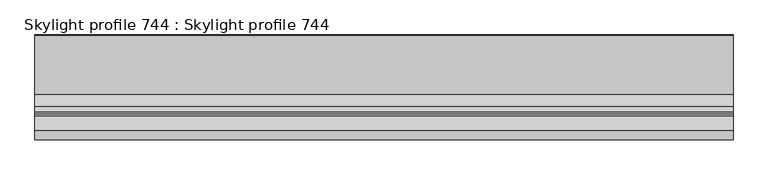
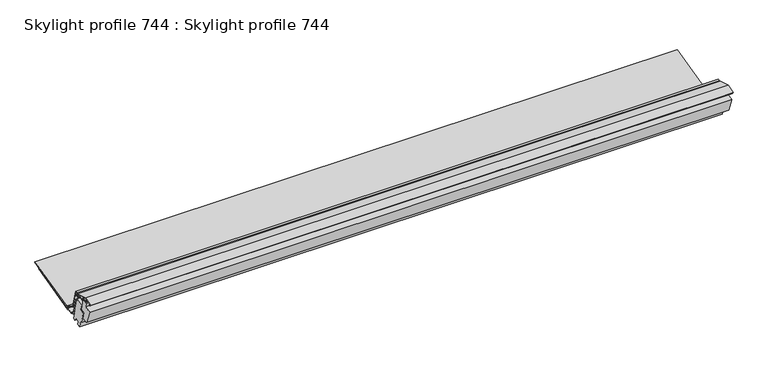
"""IFC4 building model written with IfcOpenShell, lengths in millimetres: proxy geometry, Skylight profile 744 : Skylight profile 744."""

from ifc_helpers import new_model, si_unit, frame, origin, place, context, project, spatial, polyline, outline, extrude, source, transform, mapped, element, save


def skylight_profile_744_skylight_profile_744_1989968f(model_context):
    return source(origin(), model_context, "Body", "SweptSolid", [
        extrude(outline(polyline([(10096.2573508, 43922.7064483), (10097.532491, 43917.6093806), (10110.1927133, 43920.7766051), (10113.4657593, 43918.8134908), (10115.0114469, 43912.6349746), (10131.6084885, 43916.7870784), (10137.0317176, 43914.2634297), (10139.0616447, 43910.1098329), (10137.264753, 43909.2316641), (10135.5458023, 43912.7489473), (10131.4068102, 43914.6749883), (10114.2973907, 43910.3947022), (10113.3713061, 43910.9501485), (10111.7266049, 43917.5244479), (10109.8744364, 43918.6353454), (10096.8184351, 43915.3691083), (10095.8923497, 43915.9245567), (10094.3171441, 43922.2210642), (10096.2573508, 43922.7064483)])), frame((3694.2883192, 0.0, 0.0), z_axis=(1.0, 0.0, 0.0), x_axis=(0.0, 1.0, 0.0)), (0.0, 0.0, 1.0), 2000.0),
        extrude(outline(polyline([(10079.242927, 43916.6221925), (10076.0312489, 43915.6964689), (10070.3693011, 43922.1990472), (10096.8276113, 43930.3081292), (10140.044925, 43917.228695), (10143.8105165, 43907.064565), (10138.5810742, 43903.9384198), (10137.5548647, 43905.6550718), (10141.3576537, 43907.9283678), (10138.5146506, 43915.6022359), (10096.8312865, 43928.2174303), (10073.9003145, 43921.1894255), (10076.7023802, 43917.9713366), (10078.6890046, 43918.5439547), (10079.242927, 43916.6221925)])), frame((3694.2883192, 0.0, 0.0), z_axis=(1.0, 0.0, 0.0), x_axis=(0.0, 1.0, 0.0)), (0.0, 0.0, 1.0), 2000.0),
        extrude(outline(polyline([(10145.985181, 43916.620671), (10151.5395078, 43918.0102043), (10165.844379, 43860.8299046), (10200.5304181, 43840.4836582), (10370.7180003, 43881.8704659), (10371.1905938, 43879.927104), (10200.2165946, 43838.3490527), (10164.1080064, 43859.5297424), (10150.0846852, 43915.5846135), (10148.412109, 43915.1661829), (10150.5052335, 43906.8238331), (10148.5653616, 43906.3371125), (10145.985181, 43916.620671)])), frame((3694.2883192, 0.0, 0.0), z_axis=(1.0, 0.0, 0.0), x_axis=(0.0, 1.0, 0.0)), (0.0, 0.0, 1.0), 2000.0),
        extrude(outline(polyline([(10194.6501599, 43830.8599821), (10192.6334981, 43834.9408699), (10176.4964673, 43831.2231764), (10162.6063897, 43836.4479074), (10149.394688, 43889.2597364), (10151.3348974, 43889.74511), (10164.2920903, 43837.9506423), (10176.6356497, 43833.3076316), (10193.7257878, 43837.2449047), (10195.7260908, 43833.1971203), (10350.9375941, 43872.6548936), (10351.4303591, 43870.7165482), (10194.6501599, 43830.8599821)])), frame((3694.2883192, 0.0, 0.0), z_axis=(1.0, 0.0, 0.0), x_axis=(0.0, 1.0, 0.0)), (0.0, 0.0, 1.0), 2000.0),
        extrude(outline(polyline([(10156.2334346, 43820.5271586), (10149.2528163, 43831.0794667), (10137.2155603, 43828.0680904), (10139.1867552, 43817.2760241), (10129.8324627, 43814.9063018), (10124.2729101, 43837.129283), (10118.717164, 43835.7393946), (10109.6828906, 43871.8517409), (10123.5722524, 43875.3264609), (10119.6342367, 43891.0677364), (10144.6350908, 43897.3222331), (10155.6384747, 43853.338722), (10154.7125446, 43853.1070809), (10162.472623, 43822.0880246), (10156.2334346, 43820.5271586)])), frame((3694.2883192, 0.0, 0.0), z_axis=(1.0, 0.0, 0.0), x_axis=(0.0, 1.0, 0.0)), (0.0, 0.0, 1.0), 2000.0),
        extrude(outline(polyline([(10119.2566248, 43878.3792301), (10105.7016033, 43874.747173), (10110.7413045, 43854.6029382), (10094.4955764, 43850.538723), (10092.6158882, 43851.5362563), (10076.658138, 43895.2717658), (10097.9551596, 43900.5996699), (10094.5962634, 43914.0260537), (10109.4115847, 43917.7324222), (10119.2566248, 43878.3792301)])), frame((3694.2883192, 0.0, 0.0), z_axis=(1.0, 0.0, 0.0), x_axis=(0.0, 1.0, 0.0)), (0.0, 0.0, 1.0), 2000.0),
    ])


if __name__ == "__main__":
    model = new_model("IFC4")
    model_context = context("Model", 3, world=origin())
    ifc_project = project(units=[si_unit("LENGTHUNIT", "METRE", prefix="MILLI")], contexts=[model_context])
    site = spatial("IfcSite", under=ifc_project)
    building = spatial("IfcBuilding", under=site)
    placement = place(None, origin())
    skylight_profile_744_skylight_profile_744_shape = skylight_profile_744_skylight_profile_744_1989968f(model_context)
    element("IfcBuildingElementProxy", 1, Name="Skylight profile 744 : Skylight profile 744", ObjectType="Skylight profile 744 : Skylight profile 744", at=placement, inside=building, context=model_context, shape_type="MappedRepresentation", body=[
        mapped(skylight_profile_744_skylight_profile_744_shape, transform((0.0, 0.0, 0.0), x_axis=(1.0, 0.0, 0.0), y_axis=(0.0, 1.0, 0.0), z_axis=(0.0, 0.0, 1.0))),
    ])
    save(model, "model.ifc")

# Revit data of these elements
# Type "Skylight profile 744 : Skylight profile 744"
#   NameOverride = "Skylight profile"
# Element 1 (IfcBuildingElementProxy, "Skylight profile 744 : Skylight profile 744")
#   Materials on its faces: "IfcSurfaceStyle #734"
# Materials
#   "IfcSurfaceStyle #734": class "Unassigned", colour RGB 169 181 186, transparency 0
